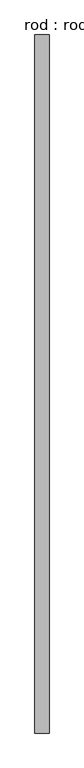
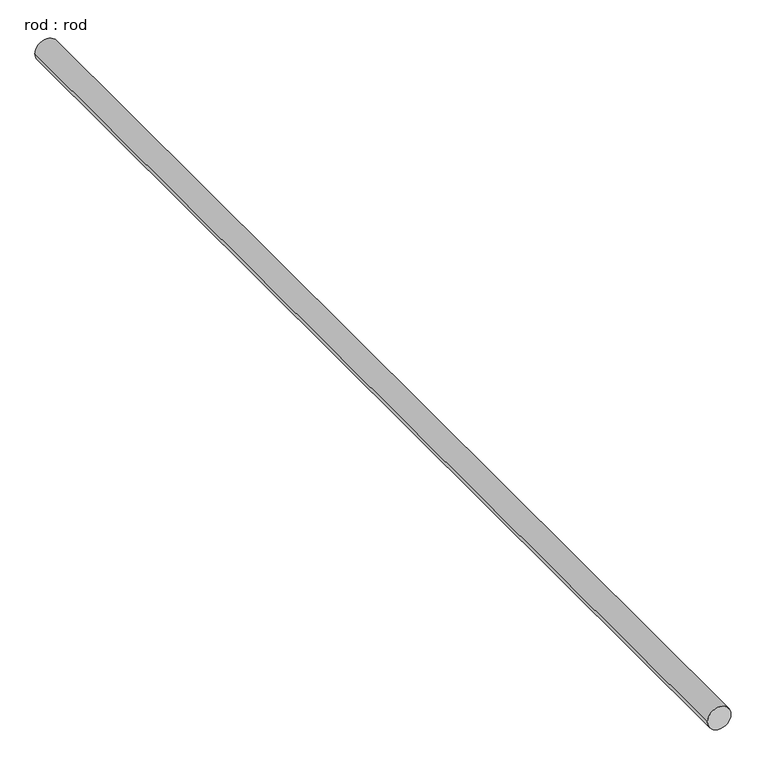
"""IFC4 building model written with IfcOpenShell, lengths in millimetres: proxy geometry, rod : rod."""

from ifc_helpers import new_model, si_unit, point, frame, frame_2d, origin, place, context, project, spatial, circle_curve, trimmed, segment, composite_curve, outline, extrude, source, transform, mapped, element, save


def rod_rod_2d8b23fc(model_context):
    return source(origin(), model_context, "Body", "SweptSolid", [
        extrude(outline(composite_curve([segment(trimmed(circle_curve(frame_2d((0.0108462, 0.0)), 200.0), [point((0.0108462, 200.0))], [point((0.0108462, -200.0))], False, "CARTESIAN"), True, "CONTINUOUS"), segment(trimmed(circle_curve(frame_2d((0.0108462, 0.0)), 200.0), [point((0.0108462, -200.0))], [point((0.0108462, 200.0))], False, "CARTESIAN"), True, "CONTINUOUS")], self_intersect=False)), frame((0.0, -5796.1602736, 0.0), z_axis=(0.0, 1.0, 0.0), x_axis=(0.0, 0.0, 1.0)), (0.0, 0.0, 1.0), 19777.7777778),
    ])


if __name__ == "__main__":
    model = new_model("IFC4")
    model_context = context("Model", 3, world=origin())
    ifc_project = project(units=[si_unit("LENGTHUNIT", "METRE", prefix="MILLI")], contexts=[model_context])
    site = spatial("IfcSite", under=ifc_project)
    building = spatial("IfcBuilding", under=site)
    placement = place(None, origin())
    rod_rod_shape = rod_rod_2d8b23fc(model_context)
    element("IfcBuildingElementProxy", 1, Name="rod : rod", ObjectType="rod : rod", at=placement, inside=building, context=model_context, shape_type="MappedRepresentation", body=[
        mapped(rod_rod_shape, transform((0.0, 0.0, 0.0), x_axis=(1.0, 0.0, 0.0), y_axis=(0.0, 1.0, 0.0), z_axis=(0.0, 0.0, 1.0))),
    ])
    save(model, "model.ifc")

# Revit data of these elements
# Type "rod : rod"
#   Default Elevation = 0
